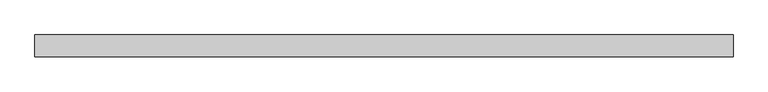
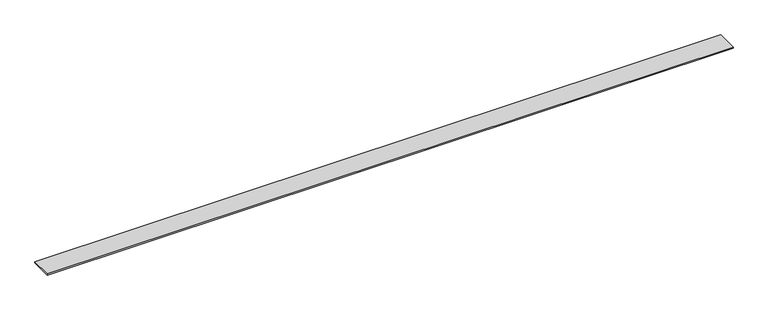
"""IFC4 building model written with IfcOpenShell, lengths in millimetres: proxy geometry, Generic Models 7:Generic Models 1:1:Generic Models 1:1 : Generic Models 7:Generic Models 1:337419:3 : Generic Models 7:Generic Models 1:1:Generic Models 1:1 : Generic Models 7:Generic Models 1:337419:306201."""

from ifc_helpers import new_model, si_unit, frame, origin, place, context, project, spatial, polyline, outline, extrude, source, transform, mapped, element, save


def generic_models_b8110da4(model_context):
    return source(origin(), model_context, "Body", "SweptSolid", [
        extrude(outline(polyline([(593719.0367239, -578841.9413841), (593719.0367239, -578918.1413841), (591280.6367239, -578918.1413841), (591280.6367239, -578841.9413841), (593719.0367239, -578841.9413841)])), frame((0.0, 0.0, 3.175), z_axis=(0.0, 0.0, 1.0), x_axis=(1.0, 0.0, 0.0)), (0.0, 0.0, 1.0), 4.7625),
    ])


if __name__ == "__main__":
    model = new_model("IFC4")
    model_context = context("Model", 3, world=origin())
    ifc_project = project(units=[si_unit("LENGTHUNIT", "METRE", prefix="MILLI")], contexts=[model_context])
    site = spatial("IfcSite", under=ifc_project)
    building = spatial("IfcBuilding", under=site)
    placement = place(None, origin())
    generic_models_shape = generic_models_b8110da4(model_context)
    element("IfcBuildingElementProxy", 1, Name="Generic Models 7:Generic Models 1:1:Generic Models 1:1 : Generic Models 7:Generic Models 1:337419:3 : Generic Models 7:Generic Models 1:1:Generic Models 1:1 : Generic Models 7:Generic Models 1:337419:306201", ObjectType="Generic Models 7:Generic Models 1:1:Generic Models 1:1 : Generic Models 7:Generic Models 1:337419:3 : Generic Models 7:Generic Models 1:1:Generic Models 1:1 : Generic Models 7:Generic Models 1:337419:306201", at=placement, inside=building, context=model_context, shape_type="MappedRepresentation", body=[
        mapped(generic_models_shape, transform((0.0, 0.0, 0.0), x_axis=(1.0, 0.0, 0.0), y_axis=(0.0, 1.0, 0.0), z_axis=(0.0, 0.0, 1.0))),
    ])
    save(model, "model.ifc")

# Revit data of these elements
# Type "Generic Models 7:Generic Models 1:1:Generic Models 1:1 : Generic Models 7:Generic Models 1:337419:3 : Generic Models 7:Generic Models 1:1:Generic Models 1:1 : Generic Models 7:Generic Models 1:337419:306201"
#   NameOverride = "Generic Models 7:Generic Models 1:1:Generic Models 1:1 : Generic Models 7:Generic Models 1:337419:306201"
#   ObjectTypeOverride = "Generic Models 1:1 : Generic Models 7:Generic Models 1:337419"
#   Reference = "Generic Models 1"
#   Tag = "306201"
# Element 1 (IfcBuildingElementProxy, "Generic Models 7:Generic Models 1:1:Generic Models 1:1 : Generic Models 7:Generic Models 1:337419:3 : Generic Models 7:Generic Models 1:1:Generic Models 1:1 : Generic Models 7:Generic Models 1:337419:306201")
#   Materials on its faces: "STAINLESS STEEL COVER PLATE"
# Materials
#   "STAINLESS STEEL COVER PLATE": class "Generic", colour RGB 190 190 190, transparency 0, Cost = 0
